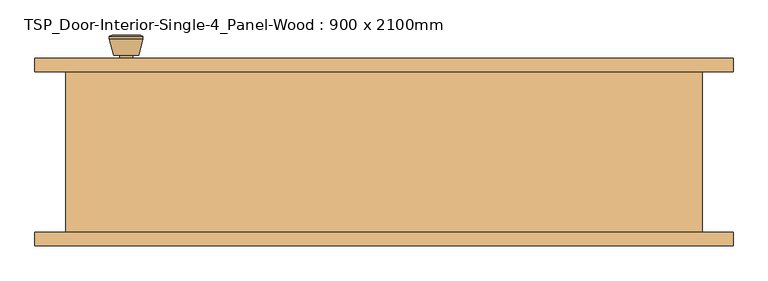
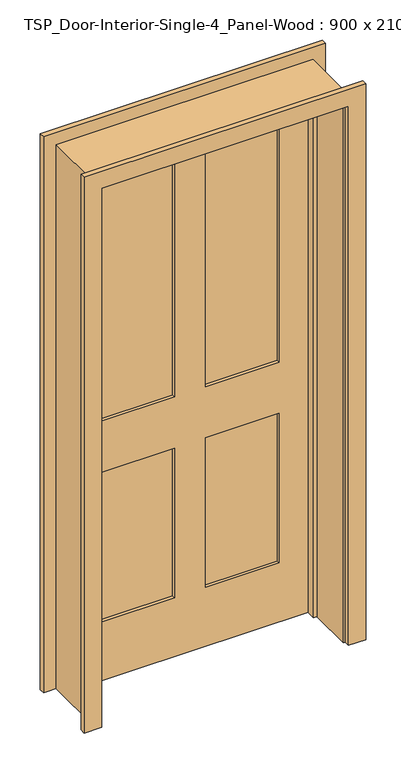
"""IFC4 building model written with IfcOpenShell, lengths in millimetres: door geometry, TSP_Door-Interior-Single-4_Panel-Wood : 900 x 2100mm."""

from ifc_helpers import new_model, si_unit, point, frame, frame_2d, origin, place, context, project, spatial, polyline, circle_curve, trimmed, segment, composite_curve, outline, extrude, faceted_brep, source, transform, mapped, element, save
from ifc_brep_helpers import plane_surface, cylinder_surface, revolved_surface, advanced_brep


def tsp_door_interior_single_4_panel_wood_900_x_2100mm_15b42963(model_context):
    return source(origin(), model_context, "Body", "SolidModel", [
        advanced_brep(
        [(-385.0, 75.825, 914.4), (-375.0, 75.825, 914.4), (-395.0, 75.825, 914.4), (-364.5241324, 26.825, 914.4), (-385.0, 26.825, 914.4), (-405.4758676, 26.825, 914.4), (-360.0, 28.6528681, 914.4), (-410.0, 28.6528681, 914.4), (-360.0, 32.1165463, 914.4), (-410.0, 32.1165463, 914.4), (-366.363764, 56.825, 914.4), (-403.636236, 56.825, 914.4), (-375.0, 56.825, 914.4), (-395.0, 56.825, 914.4)],
        [
            (0, 1),
            (1, 2, circle_curve(frame((-385.0, 75.825, 914.4), z_axis=(0.0, 1.0, 0.0), x_axis=(-1.0, 0.0, 0.0)), 10.0)),
            (2, 0),
            (2, 1, circle_curve(frame((-385.0, 75.825, 914.4), z_axis=(0.0, 1.0, 0.0), x_axis=(-1.0, 0.0, 0.0)), 10.0)),
            (3, 4),
            (4, 5),
            (5, 3, circle_curve(frame((-385.0, 26.825, 914.4), z_axis=(0.0, -1.0, 0.0), x_axis=(-1.0, 0.0, 0.0)), 20.4758676)),
            (3, 5, circle_curve(frame((-385.0, 26.825, 914.4), z_axis=(0.0, -1.0, 0.0), x_axis=(-1.0, 0.0, 0.0)), 20.4758676)),
            (6, 3),
            (5, 7),
            (7, 6, circle_curve(frame((-385.0, 28.6528681, 914.4), z_axis=(0.0, -1.0, 0.0), x_axis=(-1.0, 0.0, 0.0)), 25.0)),
            (6, 7, circle_curve(frame((-385.0, 28.6528681, 914.4), z_axis=(0.0, -1.0, 0.0), x_axis=(-1.0, 0.0, 0.0)), 25.0)),
            (8, 6),
            (7, 9),
            (9, 8, circle_curve(frame((-385.0, 32.1165463, 914.4), z_axis=(0.0, -1.0, 0.0), x_axis=(-1.0, 0.0, 0.0)), 25.0)),
            (8, 9, circle_curve(frame((-385.0, 32.1165463, 914.4), z_axis=(0.0, -1.0, 0.0), x_axis=(-1.0, 0.0, 0.0)), 25.0)),
            (10, 8),
            (9, 11),
            (11, 10, circle_curve(frame((-385.0, 56.825, 914.4), z_axis=(0.0, -1.0, 0.0), x_axis=(-1.0, 0.0, 0.0)), 18.636236)),
            (10, 11, circle_curve(frame((-385.0, 56.825, 914.4), z_axis=(0.0, -1.0, 0.0), x_axis=(-1.0, 0.0, 0.0)), 18.636236)),
            (12, 10),
            (11, 13),
            (13, 12, circle_curve(frame((-385.0, 56.825, 914.4), z_axis=(0.0, -1.0, 0.0), x_axis=(-1.0, 0.0, 0.0)), 10.0)),
            (12, 13, circle_curve(frame((-385.0, 56.825, 914.4), z_axis=(0.0, -1.0, 0.0), x_axis=(-1.0, 0.0, 0.0)), 10.0)),
            (1, 12),
            (13, 2),
        ],
        [
            plane_surface(frame((-385.0, 75.825, 914.4), z_axis=(0.0, 1.0, 0.0), x_axis=(-1.0, 0.0, 0.0))),
            plane_surface(frame((-385.0, 26.825, 914.4), z_axis=(0.0, -1.0, 0.0), x_axis=(-1.0, 0.0, 0.0))),
            revolved_surface(polyline([(-405.4758676, 26.825, 914.4), (-410.0, 28.6528681, 914.4)]), (-385.0, 75.825, 914.4), (0.0, 1.0, 0.0)),
            cylinder_surface(frame((-385.0, 75.825, 914.4), z_axis=(0.0, 1.0, 0.0), x_axis=(-1.0, 0.0, 0.0)), 25.0),
            revolved_surface(polyline([(-410.0, 32.1165463, 914.4), (-403.636236, 56.825, 914.4)]), (-385.0, 75.825, 914.4), (0.0, 1.0, 0.0)),
            plane_surface(frame((-385.0, 56.825, 914.4), z_axis=(0.0, 1.0, 0.0), x_axis=(-1.0, 0.0, 0.0))),
            cylinder_surface(frame((-385.0, 75.825, 914.4), z_axis=(0.0, 1.0, 0.0), x_axis=(-1.0, 0.0, 0.0)), 10.0),
        ],
        [
            (0, [[1, 2, 3]]),
            (0, [[-3, 4, -1]]),
            (1, [[5, 6, 7]]),
            (1, [[-6, -5, 8]]),
            (2, [[9, -7, 10, 11]]),
            (2, [[-10, -8, -9, 12]]),
            (3, [[13, -11, 14, 15]]),
            (3, [[-14, -12, -13, 16]]),
            (4, [[17, -15, 18, 19]]),
            (4, [[-18, -16, -17, 20]]),
            (5, [[21, -19, 22, 23]]),
            (5, [[-22, -20, -21, 24]]),
            (6, [[25, -23, 26, -2]]),
            (6, [[-26, -24, -25, -4]]),
        ],
    ),
        extrude(outline(composite_curve([segment(trimmed(circle_curve(frame_2d((914.4, -385.0)), 30.0), [point((914.4, -415.0))], [point((914.4, -355.0))], False, "CARTESIAN"), True, "CONTINUOUS"), segment(trimmed(circle_curve(frame_2d((914.4, -385.0)), 30.0), [point((914.4, -355.0))], [point((914.4, -415.0))], False, "CARTESIAN"), True, "CONTINUOUS")], self_intersect=False)), frame((0.0, 75.825, 0.0), z_axis=(0.0, 1.0, 0.0), x_axis=(0.0, 0.0, 1.0)), (0.0, 0.0, 1.0), 6.0),
        advanced_brep(
        [(-385.0, 122.825, 914.4), (-395.0, 122.825, 914.4), (-375.0, 122.825, 914.4), (-364.5241324, 171.825, 914.4), (-405.4758676, 171.825, 914.4), (-385.0, 171.825, 914.4), (-360.0, 169.9971319, 914.4), (-410.0, 169.9971319, 914.4), (-360.0, 166.5334537, 914.4), (-410.0, 166.5334537, 914.4), (-366.363764, 141.825, 914.4), (-403.636236, 141.825, 914.4), (-375.0, 141.825, 914.4), (-395.0, 141.825, 914.4)],
        [
            (0, 1),
            (1, 2, circle_curve(frame((-385.0, 122.825, 914.4), z_axis=(0.0, -1.0, 0.0), x_axis=(-1.0, 0.0, 0.0)), 10.0)),
            (2, 0),
            (2, 1, circle_curve(frame((-385.0, 122.825, 914.4), z_axis=(0.0, -1.0, 0.0), x_axis=(-1.0, 0.0, 0.0)), 10.0)),
            (3, 4, circle_curve(frame((-385.0, 171.825, 914.4), z_axis=(0.0, 1.0, 0.0), x_axis=(-1.0, 0.0, 0.0)), 20.4758676)),
            (4, 5),
            (5, 3),
            (4, 3, circle_curve(frame((-385.0, 171.825, 914.4), z_axis=(0.0, 1.0, 0.0), x_axis=(-1.0, 0.0, 0.0)), 20.4758676)),
            (6, 7, circle_curve(frame((-385.0, 169.9971319, 914.4), z_axis=(0.0, 1.0, 0.0), x_axis=(-1.0, 0.0, 0.0)), 25.0)),
            (7, 4),
            (3, 6),
            (7, 6, circle_curve(frame((-385.0, 169.9971319, 914.4), z_axis=(0.0, 1.0, 0.0), x_axis=(-1.0, 0.0, 0.0)), 25.0)),
            (8, 9, circle_curve(frame((-385.0, 166.5334537, 914.4), z_axis=(0.0, 1.0, 0.0), x_axis=(-1.0, 0.0, 0.0)), 25.0)),
            (9, 7),
            (6, 8),
            (9, 8, circle_curve(frame((-385.0, 166.5334537, 914.4), z_axis=(0.0, 1.0, 0.0), x_axis=(-1.0, 0.0, 0.0)), 25.0)),
            (10, 11, circle_curve(frame((-385.0, 141.825, 914.4), z_axis=(0.0, 1.0, 0.0), x_axis=(-1.0, 0.0, 0.0)), 18.636236)),
            (11, 9),
            (8, 10),
            (11, 10, circle_curve(frame((-385.0, 141.825, 914.4), z_axis=(0.0, 1.0, 0.0), x_axis=(-1.0, 0.0, 0.0)), 18.636236)),
            (12, 13, circle_curve(frame((-385.0, 141.825, 914.4), z_axis=(0.0, 1.0, 0.0), x_axis=(-1.0, 0.0, 0.0)), 10.0)),
            (13, 11),
            (10, 12),
            (13, 12, circle_curve(frame((-385.0, 141.825, 914.4), z_axis=(0.0, 1.0, 0.0), x_axis=(-1.0, 0.0, 0.0)), 10.0)),
            (1, 13),
            (12, 2),
        ],
        [
            plane_surface(frame((-385.0, 122.825, 914.4), z_axis=(0.0, -1.0, 0.0), x_axis=(-1.0, 0.0, 0.0))),
            plane_surface(frame((-385.0, 171.825, 914.4), z_axis=(0.0, 1.0, 0.0), x_axis=(-1.0, 0.0, 0.0))),
            revolved_surface(polyline([(-405.4758676, 171.825, 914.4), (-410.0, 169.9971319, 914.4)]), (-385.0, 122.825, 914.4), (0.0, -1.0, 0.0)),
            cylinder_surface(frame((-385.0, 122.825, 914.4), z_axis=(0.0, -1.0, 0.0), x_axis=(-1.0, 0.0, 0.0)), 25.0),
            revolved_surface(polyline([(-410.0, 166.5334537, 914.4), (-403.636236, 141.825, 914.4)]), (-385.0, 122.825, 914.4), (0.0, -1.0, 0.0)),
            plane_surface(frame((-385.0, 141.825, 914.4), z_axis=(0.0, -1.0, 0.0), x_axis=(-1.0, 0.0, 0.0))),
            cylinder_surface(frame((-385.0, 122.825, 914.4), z_axis=(0.0, -1.0, 0.0), x_axis=(-1.0, 0.0, 0.0)), 10.0),
        ],
        [
            (0, [[1, 2, 3]]),
            (0, [[-3, 4, -1]]),
            (1, [[5, 6, 7]]),
            (1, [[8, -7, -6]]),
            (2, [[9, 10, -5, 11]]),
            (2, [[12, -11, -8, -10]]),
            (3, [[13, 14, -9, 15]]),
            (3, [[16, -15, -12, -14]]),
            (4, [[17, 18, -13, 19]]),
            (4, [[20, -19, -16, -18]]),
            (5, [[21, 22, -17, 23]]),
            (5, [[24, -23, -20, -22]]),
            (6, [[-2, 25, -21, 26]]),
            (6, [[-4, -26, -24, -25]]),
        ],
    ),
        extrude(outline(composite_curve([segment(trimmed(circle_curve(frame_2d((914.4, -385.0)), 30.0), [point((914.4, -415.0))], [point((914.4, -355.0))], False, "CARTESIAN"), True, "CONTINUOUS"), segment(trimmed(circle_curve(frame_2d((914.4, -385.0)), 30.0), [point((914.4, -355.0))], [point((914.4, -415.0))], False, "CARTESIAN"), True, "CONTINUOUS")], self_intersect=False)), frame((0.0, 116.825, 0.0), z_axis=(0.0, 1.0, 0.0), x_axis=(0.0, 0.0, 1.0)), (0.0, 0.0, 1.0), 6.0),
        faceted_brep([(475.0, 116.825, 0.0), (475.0, -123.175, 0.0), (450.0, -123.175, 0.0), (450.0, 46.9, 0.0), (437.3, 46.9, 0.0), (437.3, 81.825, 0.0), (450.0, 81.825, 0.0), (450.0, 116.825, 0.0), (475.0, 116.825, 2125.0), (475.0, -123.175, 2125.0), (-475.0, -123.175, 2125.0), (-475.0, -123.175, 0.0), (-450.0, -123.175, 0.0), (-450.0, -123.175, 2100.0), (450.0, -123.175, 2100.0), (450.0, 46.9, 2100.0), (-450.0, 46.9, 2100.0), (-450.0, 46.9, 0.0), (-437.3, 46.9, 0.0), (-437.3, 46.9, 2087.3), (437.3, 46.9, 2087.3), (437.3, 81.825, 2087.3), (-437.3, 81.825, 2087.3), (-437.3, 81.825, 0.0), (-450.0, 81.825, 0.0), (-450.0, 81.825, 2100.0), (450.0, 81.825, 2100.0), (450.0, 116.825, 2100.0), (-450.0, 116.825, 2100.0), (-450.0, 116.825, 0.0), (-475.0, 116.825, 0.0), (-475.0, 116.825, 2125.0)], [[[0, 1, 2, 3, 4, 5, 6, 7]], [[1, 0, 8, 9]], [[2, 1, 9, 10, 11, 12, 13, 14]], [[3, 2, 14, 15]], [[4, 3, 15, 16, 17, 18, 19, 20]], [[5, 4, 20, 21]], [[6, 5, 21, 22, 23, 24, 25, 26]], [[7, 6, 26, 27]], [[0, 7, 27, 28, 29, 30, 31, 8]], [[9, 8, 31, 10]], [[15, 14, 13, 16]], [[21, 20, 19, 22]], [[27, 26, 25, 28]], [[30, 29, 24, 23, 18, 17, 12, 11]], [[10, 31, 30, 11]], [[16, 13, 12, 17]], [[22, 19, 18, 23]], [[28, 25, 24, 29]]]),
        extrude(outline(polyline([(2100.0, -450.0), (0.0, -450.0), (0.0, 450.0), (2100.0, 450.0), (2100.0, -450.0)]), holes=[polyline([(1980.0, 57.5), (1980.0, 330.0), (1014.4, 330.0), (1014.4, 57.5), (1980.0, 57.5)]), polyline([(1014.4, -57.5), (1014.4, -330.0), (1980.0, -330.0), (1980.0, -57.5), (1014.4, -57.5)]), polyline([(814.4, 57.5), (814.4, 330.0), (230.0, 330.0), (230.0, 57.5), (814.4, 57.5)]), polyline([(230.0, -57.5), (230.0, -330.0), (814.4, -330.0), (814.4, -57.5), (230.0, -57.5)])]), frame((0.0, 81.825, 0.0), z_axis=(0.0, 1.0, 0.0), x_axis=(0.0, 0.0, 1.0)), (0.0, 0.0, 1.0), 35.0),
        extrude(outline(polyline([(330.0, 93.4916667), (57.5, 93.4916667), (57.5, 105.1583333), (330.0, 105.1583333), (330.0, 93.4916667)])), frame((0.0, 0.0, 1014.4), z_axis=(0.0, 0.0, 1.0), x_axis=(1.0, 0.0, 0.0)), (0.0, 0.0, 1.0), 965.6),
        extrude(outline(polyline([(-57.5, 93.4916667), (-330.0, 93.4916667), (-330.0, 105.1583333), (-57.5, 105.1583333), (-57.5, 93.4916667)])), frame((0.0, 0.0, 1014.4), z_axis=(0.0, 0.0, 1.0), x_axis=(1.0, 0.0, 0.0)), (0.0, 0.0, 1.0), 965.6),
        extrude(outline(polyline([(330.0, 93.4916667), (57.5, 93.4916667), (57.5, 105.1583333), (330.0, 105.1583333), (330.0, 93.4916667)])), frame((0.0, 0.0, 230.0), z_axis=(0.0, 0.0, 1.0), x_axis=(1.0, 0.0, 0.0)), (0.0, 0.0, 1.0), 584.4),
        extrude(outline(polyline([(-57.5, 93.4916667), (-330.0, 93.4916667), (-330.0, 105.1583333), (-57.5, 105.1583333), (-57.5, 93.4916667)])), frame((0.0, 0.0, 230.0), z_axis=(0.0, 0.0, 1.0), x_axis=(1.0, 0.0, 0.0)), (0.0, 0.0, 1.0), 584.4),
        extrude(outline(polyline([(0.0, 456.35), (0.0, 521.35), (2171.35, 521.35), (2171.35, -521.35), (0.0, -521.35), (0.0, -456.35), (2106.35, -456.35), (2106.35, 456.35), (0.0, 456.35)])), frame((0.0, 116.825, 0.0), z_axis=(0.0, 1.0, 0.0), x_axis=(0.0, 0.0, 1.0)), (0.0, 0.0, 1.0), 20.0),
        extrude(outline(polyline([(0.0, 456.35), (0.0, 521.35), (2171.35, 521.35), (2171.35, -521.35), (0.0, -521.35), (0.0, -456.35), (2106.35, -456.35), (2106.35, 456.35), (0.0, 456.35)])), frame((0.0, -143.175, 0.0), z_axis=(0.0, 1.0, 0.0), x_axis=(0.0, 0.0, 1.0)), (0.0, 0.0, 1.0), 20.0),
    ])


if __name__ == "__main__":
    model = new_model("IFC4")
    model_context = context("Model", 3, world=origin())
    ifc_project = project(units=[si_unit("LENGTHUNIT", "METRE", prefix="MILLI")], contexts=[model_context])
    site = spatial("IfcSite", under=ifc_project)
    building = spatial("IfcBuilding", under=site)
    placement = place(None, origin())
    tsp_door_interior_single_4_panel_wood_900_x_2100mm_shape = tsp_door_interior_single_4_panel_wood_900_x_2100mm_15b42963(model_context)
    element("IfcDoor", 1, ObjectType="TSP_Door-Interior-Single-4_Panel-Wood : 900 x 2100mm", at=placement, inside=building, context=model_context, shape_type="MappedRepresentation", body=[
        mapped(tsp_door_interior_single_4_panel_wood_900_x_2100mm_shape, transform((0.0, 0.0, 0.0), x_axis=(1.0, 0.0, 0.0), y_axis=(0.0, 1.0, 0.0), z_axis=(0.0, 0.0, 1.0))),
    ])
    save(model, "model.ifc")

# Revit data of these elements
# Type "TSP_Door-Interior-Single-4_Panel-Wood : 900 x 2100mm"
#   Model = "TSP_DOOR02W"
#   Type Mark = "244"
#   Assembly Code = "C1020300"
#   Analytic Construction = "Wooden"
#   Top Rail = 120 mm
#   Thickness = 35 mm
#   Thermal Resistance (R) = 0.455703 (m²·K)/W
#   Swing Angle [instance default] = 90.00°
#   Stiles = 120 mm
#   Rough Width = 950 mm
#   Rough Height = 2125 mm
#   Mullion = 115 mm
#   Lock Rail = 200 mm
#   Height = 2100 mm
#   Width = 900 mm
#   Heat Transfer Coefficient (U) = 2.19465 W/(m²·K)
#   Bottom Rail = 230 mm
#   Define Thermal Properties by = 1
#   Trim Material = Cherry
#   Panel Material = Cherry
#   Frame Material = Cherry
#   Door Handle Material = Aluminum
#   Visual Light Transmittance = 0
#   Solar Heat Gain Coefficient = 0
#   Wall Closure = (empty or 0)
#   Function = (empty or 0)
# Element 1 (IfcDoor, "TSP_Door-Interior-Single-4_Panel-Wood : 900 x 2100mm")
#   Materials on its faces: "Cherry", "Aluminum"
# Materials
#   "Cherry": class "Wood", colour RGB 226 177 128, transparency 0, Description = "Prunus Serotina", Cost = 0
#   "Aluminum": class "Metal", colour RGB 247 247 247, transparency 0, Description = "Aluminum 6061", Cost = 0
